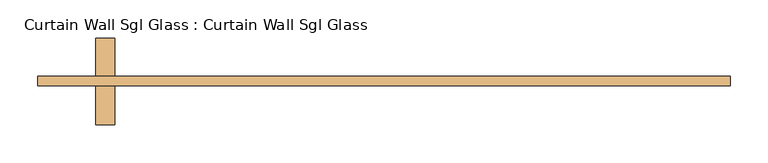
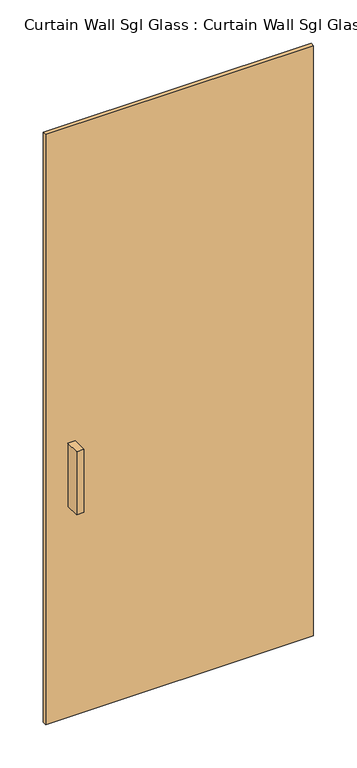
"""IFC4 building model written with IfcOpenShell, lengths in millimetres: door geometry, Curtain Wall Sgl Glass : Curtain Wall Sgl Glass."""

from ifc_helpers import new_model, si_unit, frame, origin, origin_with_axes, place, context, project, spatial, polyline, outline, extrude, source, transform, mapped, element, save


def curtain_wall_sgl_glass_curtain_wall_sgl_glass_ab2568d1(model_context):
    return source(origin(), model_context, "Body", "SweptSolid", [
        extrude(outline(polyline([(-355.6, -12.7), (-381.0, -12.7), (-381.0, 38.1), (-355.6, 38.1), (-355.6, -12.7)])), frame((0.0, 0.0, 762.0), z_axis=(0.0, 0.0, 1.0), x_axis=(1.0, 0.0, 0.0)), (0.0, 0.0, 1.0), 228.6),
        extrude(outline(polyline([(-381.0, 101.6), (-355.6, 101.6), (-355.6, 50.8), (-381.0, 50.8), (-381.0, 101.6)])), frame((0.0, 0.0, 762.0), z_axis=(0.0, 0.0, 1.0), x_axis=(1.0, 0.0, 0.0)), (0.0, 0.0, 1.0), 228.6),
        extrude(outline(polyline([(457.2, 50.8), (457.2, 38.1), (-457.2, 38.1), (-457.2, 50.8), (457.2, 50.8)])), origin_with_axes(), (0.0, 0.0, 1.0), 2133.6),
    ])


if __name__ == "__main__":
    model = new_model("IFC4")
    model_context = context("Model", 3, world=origin())
    ifc_project = project(units=[si_unit("LENGTHUNIT", "METRE", prefix="MILLI")], contexts=[model_context])
    site = spatial("IfcSite", under=ifc_project)
    building = spatial("IfcBuilding", under=site)
    placement = place(None, origin())
    curtain_wall_sgl_glass_curtain_wall_sgl_glass_shape = curtain_wall_sgl_glass_curtain_wall_sgl_glass_ab2568d1(model_context)
    element("IfcDoor", 1, ObjectType="Curtain Wall Sgl Glass : Curtain Wall Sgl Glass", at=placement, inside=building, context=model_context, shape_type="MappedRepresentation", body=[
        mapped(curtain_wall_sgl_glass_curtain_wall_sgl_glass_shape, transform((0.0, 0.0, 0.0), x_axis=(1.0, 0.0, 0.0), y_axis=(0.0, 1.0, 0.0), z_axis=(0.0, 0.0, 1.0))),
    ])
    save(model, "model.ifc")

# Revit data of these elements
# Type "Curtain Wall Sgl Glass : Curtain Wall Sgl Glass"
#   Assembly Code = "B2030100"
#   Offset = 0' - 2"
#   Function = 1
#   Handle Material = Metal - Aluminum
#   Glazing Material = Glass
# Element 1 (IfcDoor, "Curtain Wall Sgl Glass : Curtain Wall Sgl Glass")
#   Materials on its faces: "Metal - Aluminum", "Glass"
# Materials
#   "Metal - Aluminum": class "Metal", colour RGB 140 140 140, transparency 0
#   "Glass": class "Glass", colour RGB 0 128 192, transparency 0.75
